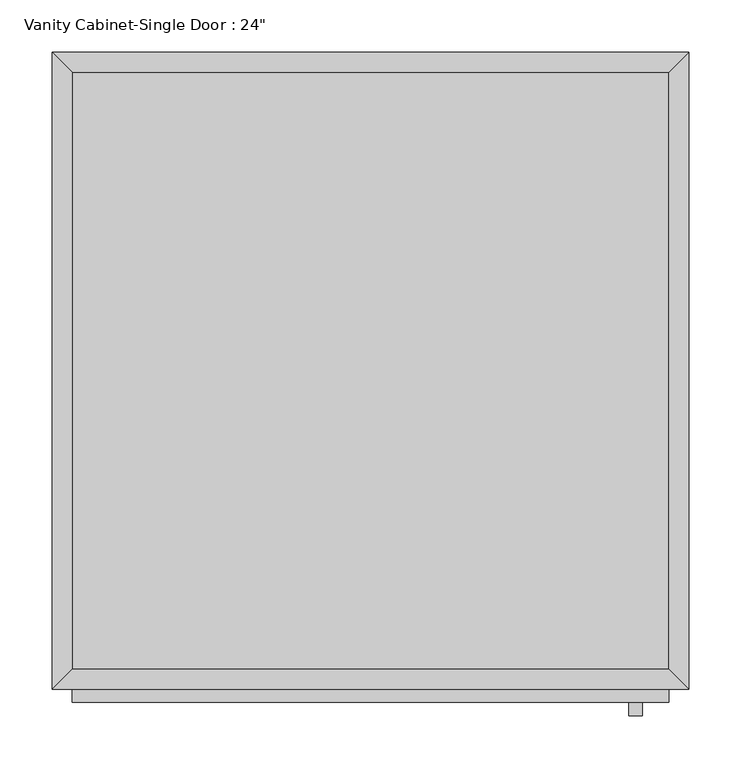
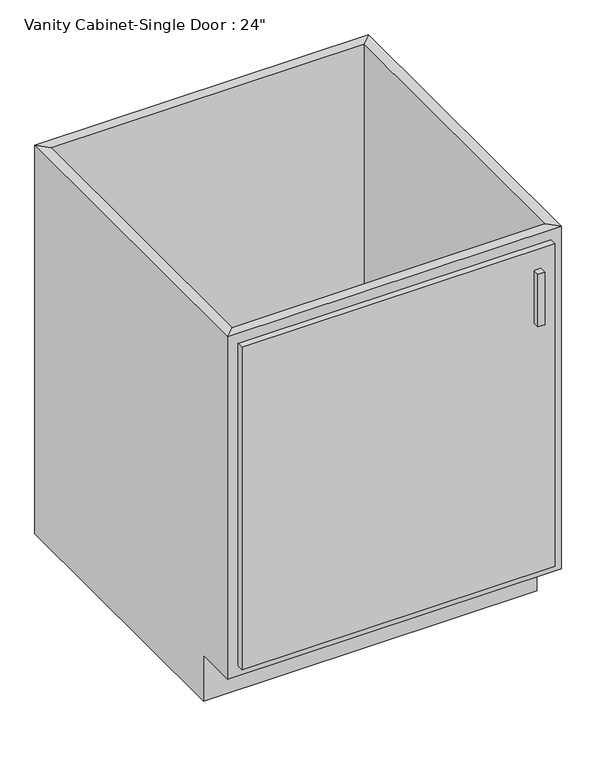
"""IFC4 building model written with IfcOpenShell, lengths in millimetres: furniture geometry."""

from ifc_helpers import new_model, si_unit, frame, origin, place, context, project, spatial, polyline, outline, extrude, faceted_brep, source, transform, mapped, element, save


def furniture_9975546c(model_context):
    return source(origin(), model_context, "Body", "SolidModel", [
        faceted_brep([(-267.0122951, -533.4, 88.9), (304.4877049, -533.4, 88.9), (304.4877049, -19.05, 88.9), (-267.0122951, -19.05, 88.9), (323.5377049, 0.0, 0.0), (323.5377049, -533.4, 0.0), (-286.0622951, -533.4, 0.0), (-286.0622951, 0.0, 0.0), (-286.0622951, 0.0, 749.3), (323.5377049, 0.0, 749.3), (-286.0622951, -533.4, 88.9), (-286.0622951, -609.6, 88.9), (-286.0622951, -609.6, 749.3), (323.5377049, -533.4, 88.9), (323.5377049, -609.6, 749.3), (323.5377049, -609.6, 88.9), (304.4877049, -590.55, 749.3), (304.4877049, -590.55, 88.9), (-267.0122951, -590.55, 88.9), (-267.0122951, -590.55, 749.3), (-267.0122951, -19.05, 749.3), (304.4877049, -19.05, 749.3)], [[[0, 1, 2, 3]], [[4, 5, 6, 7]], [[4, 7, 8, 9]], [[8, 7, 6, 10, 11, 12]], [[6, 5, 13, 1, 0, 10]], [[5, 4, 9, 14, 15, 13]], [[16, 17, 18, 19]], [[16, 19, 12, 14]], [[14, 12, 11, 15]], [[18, 17, 15, 11]], [[19, 18, 0, 3, 20]], [[12, 19, 20, 8]], [[18, 11, 10, 0]], [[20, 3, 2, 21]], [[8, 20, 21, 9]], [[17, 16, 21, 2, 1]], [[16, 14, 9, 21]], [[15, 17, 1, 13]]]),
        extrude(outline(polyline([(304.4877049, -19.05), (304.4877049, -590.55), (-267.0122951, -590.55), (-267.0122951, -19.05), (304.4877049, -19.05)])), frame((0.0, 0.0, 88.9), z_axis=(0.0, 0.0, 1.0), x_axis=(1.0, 0.0, 0.0)), (0.0, 0.0, 1.0), 19.05),
        extrude(outline(polyline([(304.4877049, -622.3), (-267.0122951, -622.3), (-267.0122951, -609.6), (304.4877049, -609.6), (304.4877049, -622.3)])), frame((0.0, 0.0, 107.95), z_axis=(0.0, 0.0, 1.0), x_axis=(1.0, 0.0, 0.0)), (0.0, 0.0, 1.0), 622.3),
        extrude(outline(polyline([(279.0877049, -635.0), (266.3877049, -635.0), (266.3877049, -622.3), (279.0877049, -622.3), (279.0877049, -635.0)])), frame((0.0, 0.0, 590.55), z_axis=(0.0, 0.0, 1.0), x_axis=(1.0, 0.0, 0.0)), (0.0, 0.0, 1.0), 101.6),
    ])


if __name__ == "__main__":
    model = new_model("IFC4")
    model_context = context("Model", 3, world=origin())
    ifc_project = project(units=[si_unit("LENGTHUNIT", "METRE", prefix="MILLI")], contexts=[model_context])
    site = spatial("IfcSite", under=ifc_project)
    building = spatial("IfcBuilding", under=site)
    placement = place(None, origin())
    furniture_shape = furniture_9975546c(model_context)
    element("IfcFurniture", 1, ObjectType="Vanity Cabinet-Single Door : 24\"", at=placement, inside=building, context=model_context, shape_type="MappedRepresentation", body=[
        mapped(furniture_shape, transform((0.0, 0.0, 0.0), x_axis=(1.0, 0.0, 0.0), y_axis=(0.0, 1.0, 0.0), z_axis=(0.0, 0.0, 1.0))),
    ])
    save(model, "model.ifc")

# Revit data of these elements
# Type "Vanity Cabinet-Single Door : 24\""
#   Assembly Code = "C1030410"
#   Depth = 2' - 0"
#   Height = 2' - 5 1/2"
#   Toe Depth = 0' - 3"
#   Toe Height = 0' - 3 1/2"
#   Width = 2' - 0"
#   Cabinet Material = none
#   Drawers Material = none
#   Handle Material = Cabinets - Handles
# Element 1 (IfcFurniture, "Vanity Cabinet-Single Door : 24\"")
#   Materials on its faces: "CASEWORK", "Cabinets", "Cabinets - Handles"
# Materials
#   "Cabinets - Handles": class "Metal", colour RGB 57 57 57, transparency 0
#   "CASEWORK": class "Generic", colour RGB 181 181 181, transparency 0, Cost = 0
#   "Cabinets": class "Miscellaneous", colour RGB 249 249 249, transparency 0
